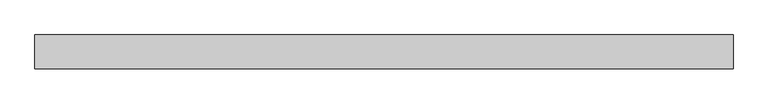
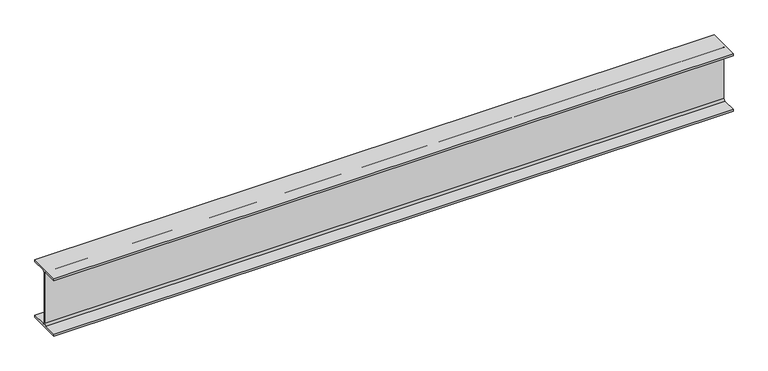
"""IFC4 building model written with IfcOpenShell, lengths in millimetres: beam geometry, Old_Steel Beam_H-KSD3502 : H_SB_ASB_H-200×200x8x12."""

from ifc_helpers import new_model, si_unit, point, frame, frame_2d, origin, place, context, project, spatial, polyline, circle_curve, trimmed, segment, composite_curve, outline, extrude, source, transform, mapped, element, save


def beam_06b2af13(model_context):
    return source(origin(), model_context, "Body", "SweptSolid", [
        extrude(outline(composite_curve([segment(polyline([(82.5, -141.5), (82.5, -151.7), (-82.5, -151.7), (-82.5, -141.5), (-11.9, -141.5)]), True, "CONTINUOUS"), segment(trimmed(circle_curve(frame_2d((-11.9, -132.6)), 8.9), [point((-11.9, -141.5))], [point((-3.0, -132.6))], True, "CARTESIAN"), True, "CONTINUOUS"), segment(polyline([(-3.0, -132.6), (-3.0, 132.6)]), True, "CONTINUOUS"), segment(trimmed(circle_curve(frame_2d((-11.9, 132.6)), 8.9), [point((-3.0, 132.6))], [point((-11.9, 141.5))], True, "CARTESIAN"), True, "CONTINUOUS"), segment(polyline([(-11.9, 141.5), (-82.5, 141.5), (-82.5, 151.7), (82.5, 151.7), (82.5, 141.5), (11.9, 141.5)]), True, "CONTINUOUS"), segment(trimmed(circle_curve(frame_2d((11.9, 132.6)), 8.9), [point((11.9, 141.5))], [point((3.0, 132.6))], True, "CARTESIAN"), True, "CONTINUOUS"), segment(polyline([(3.0, 132.6), (3.0, -132.6)]), True, "CONTINUOUS"), segment(trimmed(circle_curve(frame_2d((11.9, -132.6)), 8.9), [point((3.0, -132.6))], [point((11.9, -141.5))], True, "CARTESIAN"), True, "CONTINUOUS"), segment(polyline([(11.9, -141.5), (82.5, -141.5)]), True, "CONTINUOUS")], self_intersect=False)), frame((-1581.0252804, 0.0, 0.0), z_axis=(1.0, 0.0, 0.0), x_axis=(0.0, 1.0, 0.0)), (0.0, 0.0, 1.0), 3401.4951694),
    ])


if __name__ == "__main__":
    model = new_model("IFC4")
    model_context = context("Model", 3, world=origin())
    ifc_project = project(units=[si_unit("LENGTHUNIT", "METRE", prefix="MILLI")], contexts=[model_context])
    site = spatial("IfcSite", under=ifc_project)
    building = spatial("IfcBuilding", under=site)
    placement = place(None, origin())
    beam_shape = beam_06b2af13(model_context)
    element("IfcBeam", 1, ObjectType="Old_Steel Beam_H-KSD3502 : H_SB_ASB_H-200×200x8x12", at=placement, inside=building, context=model_context, shape_type="MappedRepresentation", body=[
        mapped(beam_shape, transform((0.0, 0.0, 0.0), x_axis=(1.0, 0.0, 0.0), y_axis=(0.0, 1.0, 0.0), z_axis=(0.0, 0.0, 1.0))),
    ])
    save(model, "model.ifc")

# Revit data of these elements
# Type "Old_Steel Beam_H-KSD3502 : H_SB_ASB_H-200×200x8x12"
#   Width = 20.0 cm
#   Web Thickness = 0.8 cm
#   Web Fillet = 1.3 cm
#   Warping Constant = 141376.0 cm⁶
#   Torsional Moment of Inertia = 26.2485 cm⁴
#   Torsional Modulus = 1.0 cm³
#   Section Area = 63.53 cm²
#   Plastic Modulus weak axis = 244.0 cm³
#   Plastic Modulus strong axis = 525.0 cm³
#   Perimeter = 1.16 m²/m
#   Nominal Weight = 49.90 kgf/m
#   Moment of Inertia weak axis = 1600.00 cm⁴
#   Moment of Inertia strong axis = 4720.00 cm⁴
#   Height = 20.0 cm
#   Flange Thickness = 1.2 cm
#   Elastic Modulus weak axis = 160.0 cm³
#   Elastic Modulus strong axis = 472.0 cm³
#   Centroid Vertical = 10.0 cm
#   Centroid Horizontal = 10.0 cm
#   Length [instance default] = 1.5240 m
#   Structural Material [instance default] = Steel, 45-345
#   Assembly Code = ""
# Element 1 (IfcBeam, "Old_Steel Beam_H-KSD3502 : H_SB_ASB_H-200×200x8x12")
#   Structural Material = none
# Materials
#   "Steel, 45-345": class "Metal", colour RGB 189 187 185, transparency 0, Description = "Steel 345 MPa", Cost = 0
